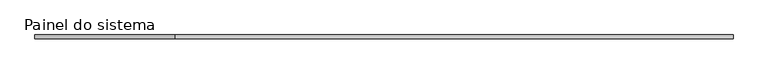
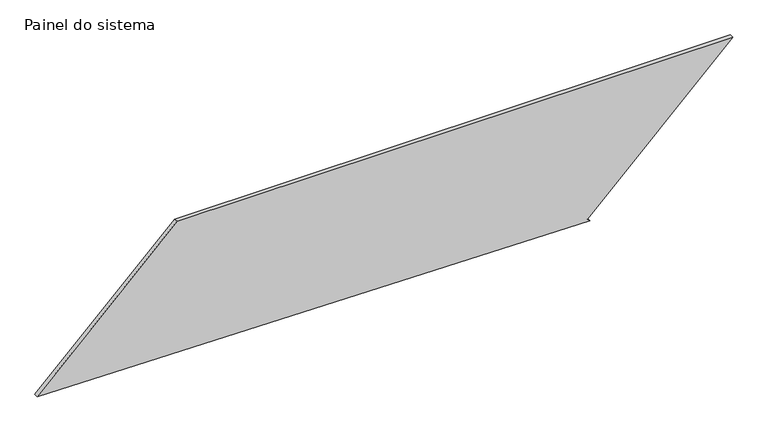
"""IFC4 building model written with IfcOpenShell, lengths in millimetres: plate geometry, Painel do sistema : Envidraçado."""

from ifc_helpers import new_model, si_unit, frame, origin, place, context, project, spatial, polyline, outline, extrude, source, transform, mapped, element, save


def painel_do_sistema_df3cb797(model_context):
    return source(origin(), model_context, "Body", "SweptSolid", [
        extrude(outline(polyline([(0.0, 1348.3545083), (17.9061609, 1330.9083224), (947.4141509, 2284.9231317), (947.4141509, -1365.7730376), (51.8752681, -2284.9231317), (0.0, 1348.3545083)])), frame((0.0, 24.5, 0.0), z_axis=(0.0, 1.0, 0.0), x_axis=(0.0, 0.0, 1.0)), (0.0, 0.0, 1.0), 25.0),
    ])


if __name__ == "__main__":
    model = new_model("IFC4")
    model_context = context("Model", 3, world=origin())
    ifc_project = project(units=[si_unit("LENGTHUNIT", "METRE", prefix="MILLI")], contexts=[model_context])
    site = spatial("IfcSite", under=ifc_project)
    building = spatial("IfcBuilding", under=site)
    placement = place(None, origin())
    painel_do_sistema_shape = painel_do_sistema_df3cb797(model_context)
    element("IfcPlate", 1, ObjectType="Painel do sistema : Envidraçado", at=placement, inside=building, context=model_context, shape_type="MappedRepresentation", body=[
        mapped(painel_do_sistema_shape, transform((0.0, 0.0, 0.0), x_axis=(1.0, 0.0, 0.0), y_axis=(0.0, 1.0, 0.0), z_axis=(0.0, 0.0, 1.0))),
    ])
    save(model, "model.ifc")

# Revit data of these elements
# Type "Painel do sistema : Envidraçado"
#   Construction Type Id = "GSP4R"
#   Analytic Construction = "Vidraça única Pilkington 1/8 pol"
#   Visual Light Transmittance = 0.9
#   Solar Heat Gain Coefficient = 0.86
#   Heat Transfer Coefficient (U) = 6.7069 W/(m²·K)
# Element 1 (IfcPlate, "Painel do sistema : Envidraçado")
#   Materials on its faces: "Vidro"
# Materials
#   "Vidro": class "Vidro", colour RGB 0 128 192, transparency 0.9, Description = "Vidro de sílica", Cost = 0
